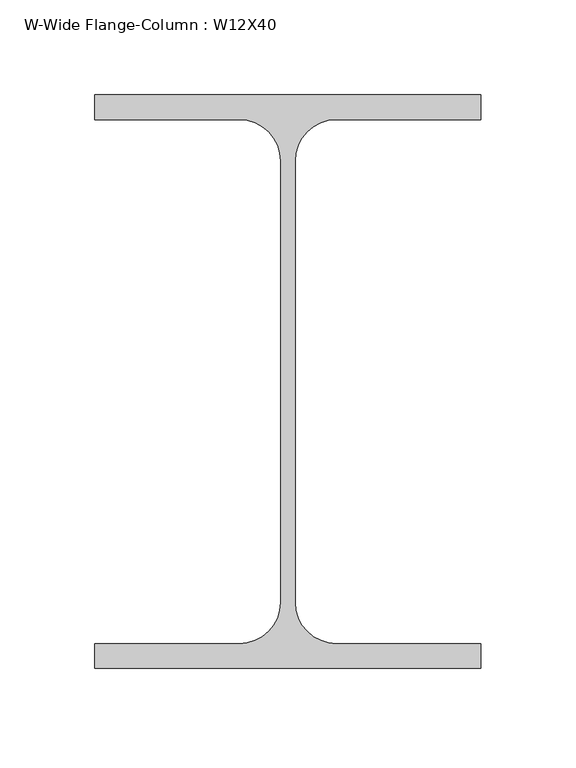
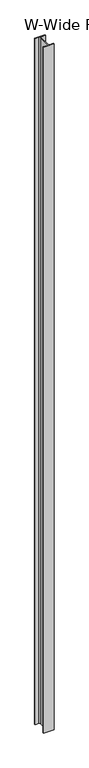
"""IFC4 building model written with IfcOpenShell, lengths in millimetres: column geometry, W-Wide Flange-Column : W12X40."""

from ifc_helpers import new_model, si_unit, point, frame, frame_2d, origin, place, context, project, spatial, polyline, circle_curve, trimmed, segment, composite_curve, outline, extrude, source, transform, mapped, element, save


def w_wide_flange_column_w12x40_01d1a46c(model_context):
    return source(origin(), model_context, "Body", "SweptSolid", [
        extrude(outline(composite_curve([segment(polyline([(101.727, 151.13), (101.727, 138.049), (25.5905, 138.049)]), True, "CONTINUOUS"), segment(trimmed(circle_curve(frame_2d((25.5905, 116.205)), 21.844), [point((25.5905, 138.049))], [point((3.7465, 116.205))], True, "CARTESIAN"), True, "CONTINUOUS"), segment(polyline([(3.7465, 116.205), (3.7465, -116.205)]), True, "CONTINUOUS"), segment(trimmed(circle_curve(frame_2d((25.5905, -116.205)), 21.844), [point((3.7465, -116.205))], [point((25.5905, -138.049))], True, "CARTESIAN"), True, "CONTINUOUS"), segment(polyline([(25.5905, -138.049), (101.727, -138.049), (101.727, -151.13), (-101.727, -151.13), (-101.727, -138.049), (-25.5905, -138.049)]), True, "CONTINUOUS"), segment(trimmed(circle_curve(frame_2d((-25.5905, -116.205)), 21.844), [point((-25.5905, -138.049))], [point((-3.7465, -116.205))], True, "CARTESIAN"), True, "CONTINUOUS"), segment(polyline([(-3.7465, -116.205), (-3.7465, 116.205)]), True, "CONTINUOUS"), segment(trimmed(circle_curve(frame_2d((-25.5905, 116.205)), 21.844), [point((-3.7465, 116.205))], [point((-25.5905, 138.049))], True, "CARTESIAN"), True, "CONTINUOUS"), segment(polyline([(-25.5905, 138.049), (-101.727, 138.049), (-101.727, 151.13), (101.727, 151.13)]), True, "CONTINUOUS")], self_intersect=False)), frame((0.0, 0.0, 13379.45), z_axis=(0.0, 0.0, 1.0), x_axis=(1.0, 0.0, 0.0)), (0.0, 0.0, 1.0), 14204.95),
    ])


if __name__ == "__main__":
    model = new_model("IFC4")
    model_context = context("Model", 3, world=origin())
    ifc_project = project(units=[si_unit("LENGTHUNIT", "METRE", prefix="MILLI")], contexts=[model_context])
    site = spatial("IfcSite", under=ifc_project)
    building = spatial("IfcBuilding", under=site)
    placement = place(None, origin())
    w_wide_flange_column_w12x40_shape = w_wide_flange_column_w12x40_01d1a46c(model_context)
    element("IfcColumn", 1, ObjectType="W-Wide Flange-Column : W12X40", at=placement, inside=building, context=model_context, shape_type="MappedRepresentation", body=[
        mapped(w_wide_flange_column_w12x40_shape, transform((0.0, 0.0, 0.0), x_axis=(1.0, 0.0, 0.0), y_axis=(0.0, 1.0, 0.0), z_axis=(0.0, 0.0, 1.0))),
    ])
    save(model, "model.ifc")

# Revit data of these elements
# Type "W-Wide Flange-Column : W12X40"
#   Assembly Code = "B10"
#   W = 40
#   bf = 0' - 8.01"
#   d = 0' - 11.9"
#   k = 0' - 1 3/8"
#   kr = 0' - 0.86"
#   tf = 0' - 0.515"
#   tw = 0' - 0.295"
#   A = 0.08125 SF
#   Structural Material [instance default] = Steel ASTM A992
# Element 1 (IfcColumn, "W-Wide Flange-Column : W12X40")
#   Materials on its faces: "Steel ASTM A992"
# Materials
#   "Steel ASTM A992": class "Metal", colour RGB 199 199 199, transparency 0, Description = "Structural steel 50ksi", Cost = 0
